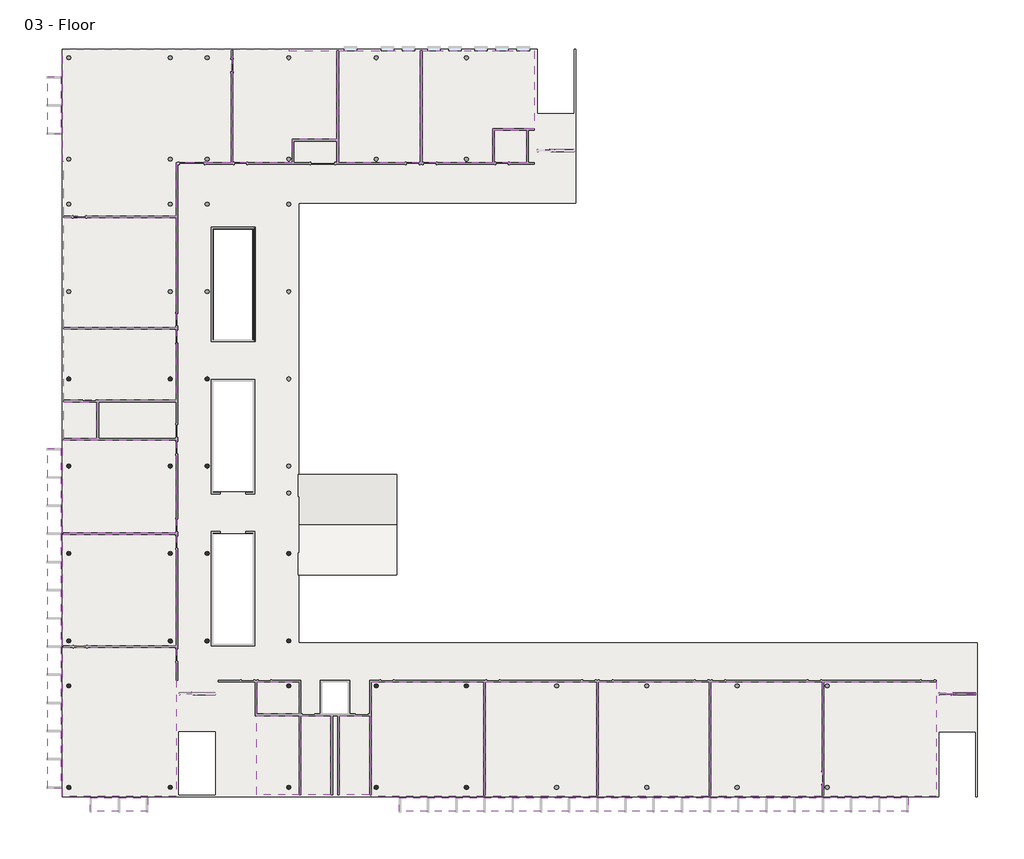
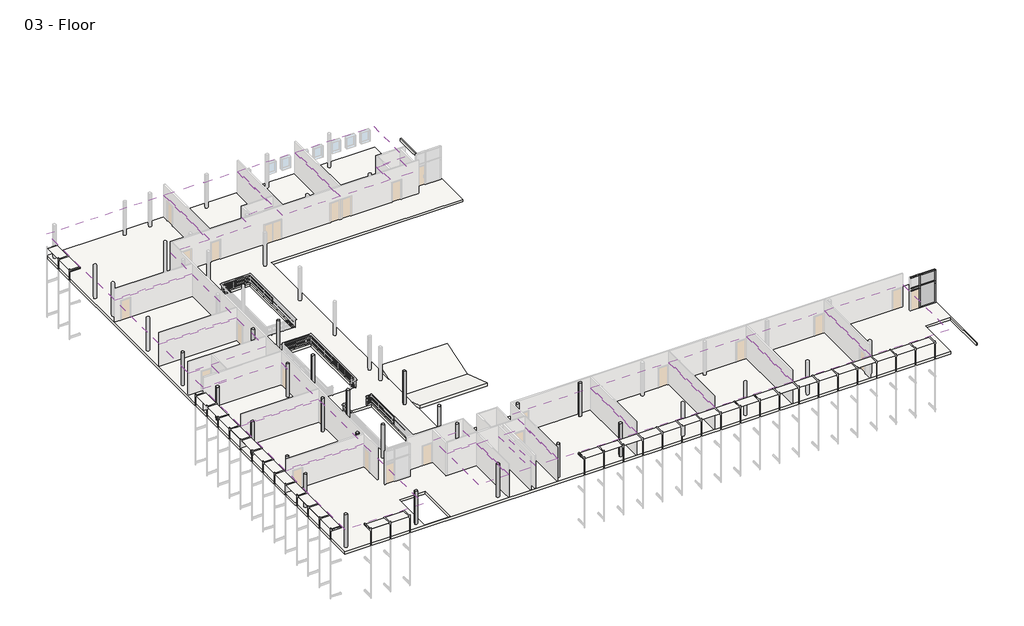
# One storey, part 3 of 4: 23 columns, 20 coverings, 14 members, 5 slabs, 2 plates, 1 roof.
"""IFC4 building model written with IfcOpenShell, lengths in millimetres."""

import ifcopenshell
import ifcopenshell.guid

model = None  # the IFC model being written
_history = None  # IfcOwnerHistory: only IFC2X3 demands one
_inside = {}  # id of a spatial element -> (the spatial element, [elements in it])
_under = {}  # id of a project, library or spatial element -> (it, [spatial elements below it])
_declared = {}  # id of a project -> (the project, [libraries it declares])
_typed = {}  # id of a type object -> (the type object, [elements of that type])
_made_of = {}  # id of a material, layer set ... -> (it, [elements and type objects made of it])


def new_model(schema):
    """Start an empty IFC model of exactly this schema.

    Asked for "IFC4X3", IfcOpenShell would pick the latest addendum, in which some entities
    have other attributes; the version numbers below select the first issue.
    IFC2X3 requires an IfcOwnerHistory on every rooted entity: one is made here for all.
    """
    global model, _history
    if schema == "IFC4X3":
        model = ifcopenshell.file(schema_version=(4, 3, 0, 0))
    else:
        model = ifcopenshell.file(schema=schema)
    _inside.clear()
    _under.clear()
    _declared.clear()
    _typed.clear()
    _made_of.clear()
    _history = None
    if model.schema == "IFC2X3":
        org = make("IfcOrganization", Name="unknown")
        user = make(
            "IfcPersonAndOrganization",
            ThePerson=make("IfcPerson", FamilyName="unknown"),
            TheOrganization=org,
        )
        app = make(
            "IfcApplication",
            ApplicationDeveloper=org,
            Version="unknown",
            ApplicationFullName="unknown",
            ApplicationIdentifier="unknown",
        )
        _history = make(
            "IfcOwnerHistory",
            OwningUser=user,
            OwningApplication=app,
            ChangeAction="ADDED",
            CreationDate=0,
        )
    return model


def make(cls, **values):
    """One entity of the class cls with the attributes given. An attribute that is None is left unset."""
    return model.create_entity(
        cls, **{name: value for name, value in values.items() if value is not None}
    )


def rooted(cls, **values):
    """An entity with a GlobalId (a new one), such as an element, a storey or a relation."""
    return make(cls, GlobalId=ifcopenshell.guid.new(), OwnerHistory=_history, **values)


def si_unit(unit_type, name, prefix=None):
    """IfcSIUnit, for example si_unit("LENGTHUNIT", "METRE", prefix="MILLI")."""
    return make("IfcSIUnit", UnitType=unit_type, Prefix=prefix, Name=name)


def assignment(units):
    """IfcUnitAssignment: the units of a project."""
    return None if units is None else make("IfcUnitAssignment", Units=units)


def point(xyz):
    """IfcCartesianPoint."""
    return None if xyz is None else make("IfcCartesianPoint", Coordinates=xyz)


def direction(xyz):
    """IfcDirection."""
    return None if xyz is None else make("IfcDirection", DirectionRatios=xyz)


def frame(location, z_axis=None, x_axis=None):
    """IfcAxis2Placement3D, a coordinate frame: its origin and axes. An axis left out is left unset."""
    return make(
        "IfcAxis2Placement3D",
        Location=point(location),
        Axis=direction(z_axis),
        RefDirection=direction(x_axis),
    )


def frame_2d(location, x_axis=None):
    """IfcAxis2Placement2D, a coordinate frame in the plane: its origin and x axis."""
    return make(
        "IfcAxis2Placement2D", Location=point(location), RefDirection=direction(x_axis)
    )


def origin():
    """The frame at (0, 0, 0) with its axes left unset."""
    return frame((0.0, 0.0, 0.0))


def place(relative_to, where):
    """IfcLocalPlacement: puts the frame where relative to a parent placement (None: the world)."""
    return make(
        "IfcLocalPlacement", PlacementRelTo=relative_to, RelativePlacement=where
    )


def context(
    kind, dimensions, precision=None, world=None, true_north=None, identifier=None
):
    """IfcGeometricRepresentationContext, for example the 3D "Model" context."""
    return make(
        "IfcGeometricRepresentationContext",
        ContextIdentifier=identifier,
        ContextType=kind,
        CoordinateSpaceDimension=dimensions,
        Precision=precision,
        WorldCoordinateSystem=world,
        TrueNorth=true_north,
    )


def project(units=None, contexts=None):
    """IfcProject with its units and contexts."""
    return rooted(
        "IfcProject",
        Name="project",
        RepresentationContexts=contexts,
        UnitsInContext=assignment(units),
    )


def spatial(cls, under=None, at=None, **own):
    """A site, building, storey or space (cls), placed at a placement, below another one or the project."""
    s = rooted(cls, ObjectPlacement=at, **own)
    if under is not None:
        _under.setdefault(under.id(), (under, []))[1].append(s)
    return s


def polyline(points):
    """IfcPolyline through the points."""
    return make("IfcPolyline", Points=[point(p) for p in points])


def circle_curve(where, radius):
    """IfcCircle in the frame where."""
    return make("IfcCircle", Position=where, Radius=radius)


def trimmed(basis, trim1, trim2, sense, master):
    """IfcTrimmedCurve: the piece of a basis curve between two trims."""
    return make(
        "IfcTrimmedCurve",
        BasisCurve=basis,
        Trim1=trim1,
        Trim2=trim2,
        SenseAgreement=sense,
        MasterRepresentation=master,
    )


def segment(curve, same_sense, transition):
    """IfcCompositeCurveSegment."""
    return make(
        "IfcCompositeCurveSegment",
        Transition=transition,
        SameSense=same_sense,
        ParentCurve=curve,
    )


def composite_curve(segments, self_intersect=None):
    """IfcCompositeCurve: segments joined end to end."""
    return make("IfcCompositeCurve", Segments=segments, SelfIntersect=self_intersect)


def outline(outer, holes=None, kind="AREA"):
    """IfcArbitraryClosedProfileDef: a profile drawn as a closed curve; with holes, ...WithVoids."""
    if holes is None:
        return make("IfcArbitraryClosedProfileDef", ProfileType=kind, OuterCurve=outer)
    return make(
        "IfcArbitraryProfileDefWithVoids",
        ProfileType=kind,
        OuterCurve=outer,
        InnerCurves=holes,
    )


def extrude(swept, where, along, depth):
    """IfcExtrudedAreaSolid: the profile swept, set in the frame where, extruded along a direction by depth."""
    return make(
        "IfcExtrudedAreaSolid",
        SweptArea=swept,
        Position=where,
        ExtrudedDirection=direction(along),
        Depth=depth,
    )


def shape(context_of_items, identifier, shape_type, items):
    """IfcShapeRepresentation: the items that make up one representation, for example the "Body"."""
    return make(
        "IfcShapeRepresentation",
        ContextOfItems=context_of_items,
        RepresentationIdentifier=identifier,
        RepresentationType=shape_type,
        Items=items,
    )


def source(mapping_origin, context_of_items, identifier, shape_type, items):
    """IfcRepresentationMap: a shape defined once, which mapped items show again and again."""
    return make(
        "IfcRepresentationMap",
        MappingOrigin=mapping_origin,
        MappedRepresentation=shape(context_of_items, identifier, shape_type, items),
    )


def transform(
    local_origin,
    x_axis=None,
    y_axis=None,
    z_axis=None,
    scale=None,
    scale2=None,
    scale3=None,
    uniform=True,
):
    """IfcCartesianTransformationOperator3D, or its non-uniform kind. x_axis, y_axis, z_axis: its Axis1, 2, 3."""
    if uniform:
        return make(
            "IfcCartesianTransformationOperator3D",
            Axis1=direction(x_axis),
            Axis2=direction(y_axis),
            LocalOrigin=point(local_origin),
            Scale=scale,
            Axis3=direction(z_axis),
        )
    return make(
        "IfcCartesianTransformationOperator3DnonUniform",
        Axis1=direction(x_axis),
        Axis2=direction(y_axis),
        LocalOrigin=point(local_origin),
        Scale=scale,
        Axis3=direction(z_axis),
        Scale2=scale2,
        Scale3=scale3,
    )


def mapped(mapping_source, mapping_target):
    """IfcMappedItem: shows the shape of a source again, moved by a transform."""
    return make(
        "IfcMappedItem", MappingSource=mapping_source, MappingTarget=mapping_target
    )


def made_of(thing, what):
    """Note that an element or type object is made of a material, layer set ...; save() writes the relation."""
    if what is not None:
        _made_of.setdefault(what.id(), (what, []))[1].append(thing)
    return thing


def element(
    cls,
    number,
    at=None,
    inside=None,
    cuts=None,
    type_object=None,
    material=None,
    context=None,
    identifier="Body",
    shape_type=None,
    held_by="IfcProductDefinitionShape",
    body=None,
    shapes=None,
    **own,
):
    """One element of the class cls, such as IfcWall. Its Tag is "e" and its number.

    at: its placement. inside: the storey or other place that contains it. cuts: it is an
    opening in that element (IfcRelVoidsElement). A single representation is given by context,
    identifier, shape_type and body (its items); several are given by shapes. held_by: the class
    of the entity that holds the representations. save() writes the other relations.
    """
    e = rooted(cls, Tag="e%d" % number, ObjectPlacement=at, **own)
    if body is not None:
        shapes = [shape(context, identifier, shape_type, body)]
    if shapes is not None:
        e.Representation = make(held_by, Representations=shapes)
    if inside is not None:
        _inside.setdefault(inside.id(), (inside, []))[1].append(e)
    if cuts is not None:
        rooted(
            "IfcRelVoidsElement", RelatingBuildingElement=cuts, RelatedOpeningElement=e
        )
    if type_object is not None:
        _typed.setdefault(type_object.id(), (type_object, []))[1].append(e)
    return made_of(e, material)


def aggregate(whole, parts):
    """IfcRelAggregates: a whole, such as a stair, and the parts it consists of."""
    return rooted("IfcRelAggregates", RelatingObject=whole, RelatedObjects=parts)


def save(model, path):
    """Write the relations noted so far, then the file.

    IfcRelAggregates (storeys below a building ...), IfcRelContainedInSpatialStructure (elements
    in a storey), IfcRelDefinesByType, IfcRelAssociatesMaterial and IfcRelDeclares: one each for
    every whole, place, type object, material and project.
    """
    for whole, parts in _under.values():
        aggregate(whole, parts)
    for where, things in _inside.values():
        rooted(
            "IfcRelContainedInSpatialStructure",
            RelatedElements=things,
            RelatingStructure=where,
        )
    for kind, things in _typed.values():
        rooted("IfcRelDefinesByType", RelatedObjects=things, RelatingType=kind)
    for what, things in _made_of.values():
        rooted("IfcRelAssociatesMaterial", RelatedObjects=things, RelatingMaterial=what)
    for by, libraries in _declared.values():
        rooted("IfcRelDeclares", RelatingContext=by, RelatedDefinitions=libraries)
    model.write(path)


def member_2b49869a(model_context):
    return source(origin(), model_context, "Body", "SweptSolid", [
        extrude(outline(polyline([(31.75, 63.5), (31.75, -63.5), (-31.75, -63.5), (-31.75, 63.5), (31.75, 63.5)])), frame((0.0, 0.0, -1219.2), z_axis=(0.0, 0.0, 1.0), x_axis=(1.0, 0.0, 0.0)), (0.0, 0.0, 1.0), 1219.2),
    ])


def member_75074519(model_context):
    return source(origin(), model_context, "Body", "SweptSolid", [
        extrude(outline(polyline([(0.0, 63.5), (0.0, -63.5), (-63.5, -63.5), (-63.5, 63.5), (0.0, 63.5)])), frame((0.0, 0.0, -1219.2), z_axis=(0.0, 0.0, 1.0), x_axis=(1.0, 0.0, 0.0)), (0.0, 0.0, 1.0), 1219.2),
    ])


def member_410c6227(model_context):
    return source(origin(), model_context, "Body", "SweptSolid", [
        extrude(outline(polyline([(31.75, 63.5), (31.75, -63.5), (-31.75, -63.5), (-31.75, 63.5), (31.75, 63.5)])), frame((0.0, 0.0, -914.4), z_axis=(0.0, 0.0, 1.0), x_axis=(1.0, 0.0, 0.0)), (0.0, 0.0, 1.0), 914.4),
    ])


def member_73c23c35(model_context):
    return source(origin(), model_context, "Body", "SweptSolid", [
        extrude(outline(polyline([(0.0, 63.5), (0.0, -63.5), (-63.5, -63.5), (-63.5, 63.5), (0.0, 63.5)])), frame((0.0, 0.0, -914.4), z_axis=(0.0, 0.0, 1.0), x_axis=(1.0, 0.0, 0.0)), (0.0, 0.0, 1.0), 914.4),
    ])


def member_6186cc23(model_context):
    return source(origin(), model_context, "Body", "SweptSolid", [
        extrude(outline(polyline([(31.75, 63.5), (31.75, -63.5), (-31.75, -63.5), (-31.75, 63.5), (31.75, 63.5)])), frame((0.0, 0.0, -2165.35), z_axis=(0.0, 0.0, 1.0), x_axis=(1.0, 0.0, 0.0)), (0.0, 0.0, 1.0), 2165.35),
    ])


def member_5d67b9fc(model_context):
    return source(origin(), model_context, "Body", "SweptSolid", [
        extrude(outline(polyline([(31.75, 63.5), (31.75, -63.5), (-31.75, -63.5), (-31.75, 63.5), (31.75, 63.5)])), frame((0.0, 0.0, -273.05), z_axis=(0.0, 0.0, 1.0), x_axis=(1.0, 0.0, 0.0)), (0.0, 0.0, 1.0), 273.05),
    ])


def member_a50b3cda(model_context):
    return source(origin(), model_context, "Body", "SweptSolid", [
        extrude(outline(polyline([(0.0, 63.5), (0.0, -63.5), (-63.5, -63.5), (-63.5, 63.5), (0.0, 63.5)])), frame((0.0, 0.0, -2165.35), z_axis=(0.0, 0.0, 1.0), x_axis=(1.0, 0.0, 0.0)), (0.0, 0.0, 1.0), 2165.35),
    ])


def member_c327c56d(model_context):
    return source(origin(), model_context, "Body", "SweptSolid", [
        extrude(outline(polyline([(0.0, 63.5), (0.0, -63.5), (-63.5, -63.5), (-63.5, 63.5), (0.0, 63.5)])), frame((0.0, 0.0, -273.05), z_axis=(0.0, 0.0, 1.0), x_axis=(1.0, 0.0, 0.0)), (0.0, 0.0, 1.0), 273.05),
    ])


def member_6c34f49c(model_context):
    return source(origin(), model_context, "Body", "SweptSolid", [
        extrude(outline(polyline([(0.0, 63.5), (0.0, -63.5), (-63.5, -63.5), (-63.5, 63.5), (0.0, 63.5)])), frame((0.0, 0.0, -285.75), z_axis=(0.0, 0.0, 1.0), x_axis=(1.0, 0.0, 0.0)), (0.0, 0.0, 1.0), 285.75),
    ])


def member_dff87739(model_context):
    return source(origin(), model_context, "Body", "SweptSolid", [
        extrude(outline(polyline([(31.75, 63.5), (31.75, -63.5), (-31.75, -63.5), (-31.75, 63.5), (31.75, 63.5)])), frame((0.0, 0.0, -285.75), z_axis=(0.0, 0.0, 1.0), x_axis=(1.0, 0.0, 0.0)), (0.0, 0.0, 1.0), 285.75),
    ])


def member_76223ac8(model_context):
    return source(origin(), model_context, "Body", "SweptSolid", [
        extrude(outline(polyline([(31.75, 63.5), (31.75, -63.5), (-31.75, -63.5), (-31.75, 63.5), (31.75, 63.5)])), frame((0.0, 0.0, -1263.65), z_axis=(0.0, 0.0, 1.0), x_axis=(1.0, 0.0, 0.0)), (0.0, 0.0, 1.0), 1263.65),
    ])


def member_e7b2e991(model_context):
    return source(origin(), model_context, "Body", "SweptSolid", [
        extrude(outline(polyline([(0.0, 63.5), (0.0, -63.5), (-63.5, -63.5), (-63.5, 63.5), (0.0, 63.5)])), frame((0.0, 0.0, -1263.65), z_axis=(0.0, 0.0, 1.0), x_axis=(1.0, 0.0, 0.0)), (0.0, 0.0, 1.0), 1263.65),
    ])


def system_panel_glazed_00df446d(model_context):
    return source(origin(), model_context, "Body", "SweptSolid", [
        extrude(outline(polyline([(0.0, -774.7), (0.0, -488.95), (0.0, 774.7), (2101.85, 774.7), (2343.15, 774.7), (2343.15, -488.95), (2343.15, -774.7), (2101.85, -774.7), (0.0, -774.7)])), frame((0.0, 19.05, 0.0), z_axis=(0.0, 1.0, 0.0), x_axis=(0.0, 0.0, 1.0)), (0.0, 0.0, 1.0), 25.4),
    ])


def system_panel_glazed_835a6d4f(model_context):
    return source(origin(), model_context, "Body", "SweptSolid", [
        extrude(outline(polyline([(0.0, -774.7), (0.0, -488.95), (0.0, 774.7), (1123.95, 774.7), (1123.95, -488.95), (1123.95, -774.7), (0.0, -774.7)])), frame((0.0, 19.05, 0.0), z_axis=(0.0, 1.0, 0.0), x_axis=(0.0, 0.0, 1.0)), (0.0, 0.0, 1.0), 25.4),
    ])


model = new_model("IFC4")

# Units and contexts
model_context = context("Model", 3, world=origin())
ifc_project = project(units=[si_unit("LENGTHUNIT", "METRE", prefix="MILLI")], contexts=[model_context])

# Site, building, storey
site = spatial("IfcSite", under=ifc_project)
building = spatial("IfcBuilding", under=site)
storey = spatial("IfcBuildingStorey", under=building, Name="03 - Floor", Elevation=7315.2)

# Columns
placement = place(None, origin())
element("IfcColumn", 1, ObjectType="Concrete-Round-Column : 12\"", at=placement, inside=storey, context=model_context, shape_type="SweptSolid", body=[
    extrude(outline(composite_curve([segment(trimmed(circle_curve(frame_2d((635.9207476, 30064.0)), 152.4), [point((788.3207476, 30064.0))], [point((483.5207476, 30064.0))], False, "CARTESIAN"), True, "CONTINUOUS"), segment(trimmed(circle_curve(frame_2d((635.9207476, 30064.0)), 152.4), [point((483.5207476, 30064.0))], [point((788.3207476, 30064.0))], False, "CARTESIAN"), True, "CONTINUOUS")], self_intersect=False)), frame((0.0, 0.0, 7315.2), z_axis=(0.0, 0.0, 1.0), x_axis=(1.0, 0.0, 0.0)), (0.0, 0.0, 1.0), 3657.6),
])
element("IfcColumn", 2, ObjectType="Concrete-Round-Column : 12\"", at=placement, inside=storey, context=model_context, shape_type="SweptSolid", body=[
    extrude(outline(composite_curve([segment(trimmed(circle_curve(frame_2d((635.9207476, 23764.8)), 152.4), [point((788.3207476, 23764.8))], [point((483.5207476, 23764.8))], False, "CARTESIAN"), True, "CONTINUOUS"), segment(trimmed(circle_curve(frame_2d((635.9207476, 23764.8)), 152.4), [point((483.5207476, 23764.8))], [point((788.3207476, 23764.8))], False, "CARTESIAN"), True, "CONTINUOUS")], self_intersect=False)), frame((0.0, 0.0, 7315.2), z_axis=(0.0, 0.0, 1.0), x_axis=(1.0, 0.0, 0.0)), (0.0, 0.0, 1.0), 3657.6),
])
element("IfcColumn", 3, ObjectType="Concrete-Round-Column : 12\"", at=placement, inside=storey, context=model_context, shape_type="SweptSolid", body=[
    extrude(outline(composite_curve([segment(trimmed(circle_curve(frame_2d((635.9207476, 17465.6)), 152.4), [point((788.3207476, 17465.6))], [point((483.5207476, 17465.6))], False, "CARTESIAN"), True, "CONTINUOUS"), segment(trimmed(circle_curve(frame_2d((635.9207476, 17465.6)), 152.4), [point((483.5207476, 17465.6))], [point((788.3207476, 17465.6))], False, "CARTESIAN"), True, "CONTINUOUS")], self_intersect=False)), frame((0.0, 0.0, 7315.2), z_axis=(0.0, 0.0, 1.0), x_axis=(1.0, 0.0, 0.0)), (0.0, 0.0, 1.0), 3657.6),
])
element("IfcColumn", 4, ObjectType="Concrete-Round-Column : 12\"", at=placement, inside=storey, context=model_context, shape_type="SweptSolid", body=[
    extrude(outline(composite_curve([segment(trimmed(circle_curve(frame_2d((635.9207476, 11166.4)), 152.4), [point((788.3207476, 11166.4))], [point((483.5207476, 11166.4))], False, "CARTESIAN"), True, "CONTINUOUS"), segment(trimmed(circle_curve(frame_2d((635.9207476, 11166.4)), 152.4), [point((483.5207476, 11166.4))], [point((788.3207476, 11166.4))], False, "CARTESIAN"), True, "CONTINUOUS")], self_intersect=False)), frame((0.0, 0.0, 7315.2), z_axis=(0.0, 0.0, 1.0), x_axis=(1.0, 0.0, 0.0)), (0.0, 0.0, 1.0), 3657.6),
])
element("IfcColumn", 5, ObjectType="Concrete-Round-Column : 12\"", at=placement, inside=storey, context=model_context, shape_type="SweptSolid", body=[
    extrude(outline(composite_curve([segment(trimmed(circle_curve(frame_2d((635.9207476, 7915.2)), 152.4), [point((788.3207476, 7915.2))], [point((483.5207476, 7915.2))], False, "CARTESIAN"), True, "CONTINUOUS"), segment(trimmed(circle_curve(frame_2d((635.9207476, 7915.2)), 152.4), [point((483.5207476, 7915.2))], [point((788.3207476, 7915.2))], False, "CARTESIAN"), True, "CONTINUOUS")], self_intersect=False)), frame((0.0, 0.0, 7315.2), z_axis=(0.0, 0.0, 1.0), x_axis=(1.0, 0.0, 0.0)), (0.0, 0.0, 1.0), 3657.6),
])
element("IfcColumn", 6, ObjectType="Concrete-Round-Column : 12\"", at=placement, inside=storey, context=model_context, shape_type="SweptSolid", body=[
    extrude(outline(composite_curve([segment(trimmed(circle_curve(frame_2d((635.9207476, 600.0)), 152.4), [point((788.3207476, 600.0))], [point((483.5207476, 600.0))], False, "CARTESIAN"), True, "CONTINUOUS"), segment(trimmed(circle_curve(frame_2d((635.9207476, 600.0)), 152.4), [point((483.5207476, 600.0))], [point((788.3207476, 600.0))], False, "CARTESIAN"), True, "CONTINUOUS")], self_intersect=False)), frame((0.0, 0.0, 7315.2), z_axis=(0.0, 0.0, 1.0), x_axis=(1.0, 0.0, 0.0)), (0.0, 0.0, 1.0), 3657.6),
])
element("IfcColumn", 7, ObjectType="Concrete-Round-Column : 12\"", at=placement, inside=storey, context=model_context, shape_type="SweptSolid", body=[
    extrude(outline(composite_curve([segment(trimmed(circle_curve(frame_2d((10592.7207476, 30064.0)), 152.4), [point((10745.1207476, 30064.0))], [point((10440.3207476, 30064.0))], False, "CARTESIAN"), True, "CONTINUOUS"), segment(trimmed(circle_curve(frame_2d((10592.7207476, 30064.0)), 152.4), [point((10440.3207476, 30064.0))], [point((10745.1207476, 30064.0))], False, "CARTESIAN"), True, "CONTINUOUS")], self_intersect=False)), frame((0.0, 0.0, 7315.2), z_axis=(0.0, 0.0, 1.0), x_axis=(1.0, 0.0, 0.0)), (0.0, 0.0, 1.0), 3657.6),
])
element("IfcColumn", 8, ObjectType="Concrete-Round-Column : 12\"", at=placement, inside=storey, context=model_context, shape_type="SweptSolid", body=[
    extrude(outline(composite_curve([segment(trimmed(circle_curve(frame_2d((10592.7207476, 23764.8)), 152.4), [point((10745.1207476, 23764.8))], [point((10440.3207476, 23764.8))], False, "CARTESIAN"), True, "CONTINUOUS"), segment(trimmed(circle_curve(frame_2d((10592.7207476, 23764.8)), 152.4), [point((10440.3207476, 23764.8))], [point((10745.1207476, 23764.8))], False, "CARTESIAN"), True, "CONTINUOUS")], self_intersect=False)), frame((0.0, 0.0, 7315.2), z_axis=(0.0, 0.0, 1.0), x_axis=(1.0, 0.0, 0.0)), (0.0, 0.0, 1.0), 3657.6),
])
element("IfcColumn", 9, ObjectType="Concrete-Round-Column : 12\"", at=placement, inside=storey, context=model_context, shape_type="SweptSolid", body=[
    extrude(outline(composite_curve([segment(trimmed(circle_curve(frame_2d((10592.7207476, 17465.6)), 152.4), [point((10745.1207476, 17465.6))], [point((10440.3207476, 17465.6))], False, "CARTESIAN"), True, "CONTINUOUS"), segment(trimmed(circle_curve(frame_2d((10592.7207476, 17465.6)), 152.4), [point((10440.3207476, 17465.6))], [point((10745.1207476, 17465.6))], False, "CARTESIAN"), True, "CONTINUOUS")], self_intersect=False)), frame((0.0, 0.0, 7315.2), z_axis=(0.0, 0.0, 1.0), x_axis=(1.0, 0.0, 0.0)), (0.0, 0.0, 1.0), 3657.6),
])
element("IfcColumn", 10, ObjectType="Concrete-Round-Column : 12\"", at=placement, inside=storey, context=model_context, shape_type="SweptSolid", body=[
    extrude(outline(composite_curve([segment(trimmed(circle_curve(frame_2d((10592.7207476, 11166.4)), 152.4), [point((10745.1207476, 11166.4))], [point((10440.3207476, 11166.4))], False, "CARTESIAN"), True, "CONTINUOUS"), segment(trimmed(circle_curve(frame_2d((10592.7207476, 11166.4)), 152.4), [point((10440.3207476, 11166.4))], [point((10745.1207476, 11166.4))], False, "CARTESIAN"), True, "CONTINUOUS")], self_intersect=False)), frame((0.0, 0.0, 7315.2), z_axis=(0.0, 0.0, 1.0), x_axis=(1.0, 0.0, 0.0)), (0.0, 0.0, 1.0), 3657.6),
])
element("IfcColumn", 11, ObjectType="Concrete-Round-Column : 12\"", at=placement, inside=storey, context=model_context, shape_type="SweptSolid", body=[
    extrude(outline(composite_curve([segment(trimmed(circle_curve(frame_2d((16485.5207476, 17465.6)), 152.4), [point((16637.9207476, 17465.6))], [point((16333.1207476, 17465.6))], False, "CARTESIAN"), True, "CONTINUOUS"), segment(trimmed(circle_curve(frame_2d((16485.5207476, 17465.6)), 152.4), [point((16333.1207476, 17465.6))], [point((16637.9207476, 17465.6))], False, "CARTESIAN"), True, "CONTINUOUS")], self_intersect=False)), frame((0.0, 0.0, 7315.2), z_axis=(0.0, 0.0, 1.0), x_axis=(1.0, 0.0, 0.0)), (0.0, 0.0, 1.0), 3657.6),
])
element("IfcColumn", 12, ObjectType="Concrete-Round-Column : 12\"", at=placement, inside=storey, context=model_context, shape_type="SweptSolid", body=[
    extrude(outline(composite_curve([segment(trimmed(circle_curve(frame_2d((16485.5207476, 11166.4)), 152.4), [point((16637.9207476, 11166.4))], [point((16333.1207476, 11166.4))], False, "CARTESIAN"), True, "CONTINUOUS"), segment(trimmed(circle_curve(frame_2d((16485.5207476, 11166.4)), 152.4), [point((16333.1207476, 11166.4))], [point((16637.9207476, 11166.4))], False, "CARTESIAN"), True, "CONTINUOUS")], self_intersect=False)), frame((0.0, 0.0, 7315.2), z_axis=(0.0, 0.0, 1.0), x_axis=(1.0, 0.0, 0.0)), (0.0, 0.0, 1.0), 3657.6),
])
element("IfcColumn", 13, ObjectType="Concrete-Round-Column : 12\"", at=placement, inside=storey, context=model_context, shape_type="SweptSolid", body=[
    extrude(outline(composite_curve([segment(trimmed(circle_curve(frame_2d((16485.5207476, 7915.2)), 152.4), [point((16637.9207476, 7915.2))], [point((16333.1207476, 7915.2))], False, "CARTESIAN"), True, "CONTINUOUS"), segment(trimmed(circle_curve(frame_2d((16485.5207476, 7915.2)), 152.4), [point((16333.1207476, 7915.2))], [point((16637.9207476, 7915.2))], False, "CARTESIAN"), True, "CONTINUOUS")], self_intersect=False)), frame((0.0, 0.0, 7315.2), z_axis=(0.0, 0.0, 1.0), x_axis=(1.0, 0.0, 0.0)), (0.0, 0.0, 1.0), 3657.6),
])
element("IfcColumn", 14, ObjectType="Concrete-Round-Column : 12\"", at=placement, inside=storey, context=model_context, shape_type="SweptSolid", body=[
    extrude(outline(composite_curve([segment(trimmed(circle_curve(frame_2d((16485.5207476, 600.0)), 152.4), [point((16637.9207476, 600.0))], [point((16333.1207476, 600.0))], False, "CARTESIAN"), True, "CONTINUOUS"), segment(trimmed(circle_curve(frame_2d((16485.5207476, 600.0)), 152.4), [point((16333.1207476, 600.0))], [point((16637.9207476, 600.0))], False, "CARTESIAN"), True, "CONTINUOUS")], self_intersect=False)), frame((0.0, 0.0, 7315.2), z_axis=(0.0, 0.0, 1.0), x_axis=(1.0, 0.0, 0.0)), (0.0, 0.0, 1.0), 3657.6),
])
element("IfcColumn", 15, ObjectType="Concrete-Round-Column : 12\"", at=placement, inside=storey, context=model_context, shape_type="SweptSolid", body=[
    extrude(outline(composite_curve([segment(trimmed(circle_curve(frame_2d((22784.7207476, 7915.2)), 152.4), [point((22937.1207476, 7915.2))], [point((22632.3207476, 7915.2))], False, "CARTESIAN"), True, "CONTINUOUS"), segment(trimmed(circle_curve(frame_2d((22784.7207476, 7915.2)), 152.4), [point((22632.3207476, 7915.2))], [point((22937.1207476, 7915.2))], False, "CARTESIAN"), True, "CONTINUOUS")], self_intersect=False)), frame((0.0, 0.0, 7315.2), z_axis=(0.0, 0.0, 1.0), x_axis=(1.0, 0.0, 0.0)), (0.0, 0.0, 1.0), 3657.6),
])
element("IfcColumn", 16, ObjectType="Concrete-Round-Column : 12\"", at=placement, inside=storey, context=model_context, shape_type="SweptSolid", body=[
    extrude(outline(composite_curve([segment(trimmed(circle_curve(frame_2d((22784.7207476, 600.0)), 152.4), [point((22937.1207476, 600.0))], [point((22632.3207476, 600.0))], False, "CARTESIAN"), True, "CONTINUOUS"), segment(trimmed(circle_curve(frame_2d((22784.7207476, 600.0)), 152.4), [point((22632.3207476, 600.0))], [point((22937.1207476, 600.0))], False, "CARTESIAN"), True, "CONTINUOUS")], self_intersect=False)), frame((0.0, 0.0, 7315.2), z_axis=(0.0, 0.0, 1.0), x_axis=(1.0, 0.0, 0.0)), (0.0, 0.0, 1.0), 3657.6),
])
element("IfcColumn", 17, ObjectType="Concrete-Round-Column : 12\"", at=placement, inside=storey, context=model_context, shape_type="SweptSolid", body=[
    extrude(outline(composite_curve([segment(trimmed(circle_curve(frame_2d((29287.1207476, 7915.2)), 152.4), [point((29439.5207476, 7915.2))], [point((29134.7207476, 7915.2))], False, "CARTESIAN"), True, "CONTINUOUS"), segment(trimmed(circle_curve(frame_2d((29287.1207476, 7915.2)), 152.4), [point((29134.7207476, 7915.2))], [point((29439.5207476, 7915.2))], False, "CARTESIAN"), True, "CONTINUOUS")], self_intersect=False)), frame((0.0, 0.0, 7315.2), z_axis=(0.0, 0.0, 1.0), x_axis=(1.0, 0.0, 0.0)), (0.0, 0.0, 1.0), 3657.6),
])
element("IfcColumn", 18, ObjectType="Concrete-Round-Column : 12\"", at=placement, inside=storey, context=model_context, shape_type="SweptSolid", body=[
    extrude(outline(composite_curve([segment(trimmed(circle_curve(frame_2d((29287.1207476, 600.0)), 152.4), [point((29439.5207476, 600.0))], [point((29134.7207476, 600.0))], False, "CARTESIAN"), True, "CONTINUOUS"), segment(trimmed(circle_curve(frame_2d((29287.1207476, 600.0)), 152.4), [point((29134.7207476, 600.0))], [point((29439.5207476, 600.0))], False, "CARTESIAN"), True, "CONTINUOUS")], self_intersect=False)), frame((0.0, 0.0, 7315.2), z_axis=(0.0, 0.0, 1.0), x_axis=(1.0, 0.0, 0.0)), (0.0, 0.0, 1.0), 3657.6),
])
element("IfcColumn", 19, ObjectType="Concrete-Round-Column : 12\"", at=placement, inside=storey, context=model_context, shape_type="SweptSolid", body=[
    extrude(outline(composite_curve([segment(trimmed(circle_curve(frame_2d((7951.1207476, 30064.0)), 152.4), [point((8103.5207476, 30064.0))], [point((7798.7207476, 30064.0))], False, "CARTESIAN"), True, "CONTINUOUS"), segment(trimmed(circle_curve(frame_2d((7951.1207476, 30064.0)), 152.4), [point((7798.7207476, 30064.0))], [point((8103.5207476, 30064.0))], False, "CARTESIAN"), True, "CONTINUOUS")], self_intersect=False)), frame((0.0, 0.0, 7315.2), z_axis=(0.0, 0.0, 1.0), x_axis=(1.0, 0.0, 0.0)), (0.0, 0.0, 1.0), 3657.6),
])
element("IfcColumn", 20, ObjectType="Concrete-Round-Column : 12\"", at=placement, inside=storey, context=model_context, shape_type="SweptSolid", body=[
    extrude(outline(composite_curve([segment(trimmed(circle_curve(frame_2d((7951.1207476, 23764.8)), 152.4), [point((8103.5207476, 23764.8))], [point((7798.7207476, 23764.8))], False, "CARTESIAN"), True, "CONTINUOUS"), segment(trimmed(circle_curve(frame_2d((7951.1207476, 23764.8)), 152.4), [point((7798.7207476, 23764.8))], [point((8103.5207476, 23764.8))], False, "CARTESIAN"), True, "CONTINUOUS")], self_intersect=False)), frame((0.0, 0.0, 7315.2), z_axis=(0.0, 0.0, 1.0), x_axis=(1.0, 0.0, 0.0)), (0.0, 0.0, 1.0), 3657.6),
])
element("IfcColumn", 21, ObjectType="Concrete-Round-Column : 12\"", at=placement, inside=storey, context=model_context, shape_type="SweptSolid", body=[
    extrude(outline(composite_curve([segment(trimmed(circle_curve(frame_2d((7951.1207476, 17465.6)), 152.4), [point((8103.5207476, 17465.6))], [point((7798.7207476, 17465.6))], False, "CARTESIAN"), True, "CONTINUOUS"), segment(trimmed(circle_curve(frame_2d((7951.1207476, 17465.6)), 152.4), [point((7798.7207476, 17465.6))], [point((8103.5207476, 17465.6))], False, "CARTESIAN"), True, "CONTINUOUS")], self_intersect=False)), frame((0.0, 0.0, 7315.2), z_axis=(0.0, 0.0, 1.0), x_axis=(1.0, 0.0, 0.0)), (0.0, 0.0, 1.0), 3657.6),
])
element("IfcColumn", 22, ObjectType="Concrete-Round-Column : 12\"", at=placement, inside=storey, context=model_context, shape_type="SweptSolid", body=[
    extrude(outline(composite_curve([segment(trimmed(circle_curve(frame_2d((7951.1207476, 11166.4)), 152.4), [point((8103.5207476, 11166.4))], [point((7798.7207476, 11166.4))], False, "CARTESIAN"), True, "CONTINUOUS"), segment(trimmed(circle_curve(frame_2d((7951.1207476, 11166.4)), 152.4), [point((7798.7207476, 11166.4))], [point((8103.5207476, 11166.4))], False, "CARTESIAN"), True, "CONTINUOUS")], self_intersect=False)), frame((0.0, 0.0, 7315.2), z_axis=(0.0, 0.0, 1.0), x_axis=(1.0, 0.0, 0.0)), (0.0, 0.0, 1.0), 3657.6),
])
element("IfcColumn", 23, ObjectType="Concrete-Round-Column : 12\"", at=placement, inside=storey, context=model_context, shape_type="SweptSolid", body=[
    extrude(outline(composite_curve([segment(trimmed(circle_curve(frame_2d((7951.1207476, 600.0)), 152.4), [point((8103.5207476, 600.0))], [point((7798.7207476, 600.0))], False, "CARTESIAN"), True, "CONTINUOUS"), segment(trimmed(circle_curve(frame_2d((7951.1207476, 600.0)), 152.4), [point((7798.7207476, 600.0))], [point((8103.5207476, 600.0))], False, "CARTESIAN"), True, "CONTINUOUS")], self_intersect=False)), frame((0.0, 0.0, 7315.2), z_axis=(0.0, 0.0, 1.0), x_axis=(1.0, 0.0, 0.0)), (0.0, 0.0, 1.0), 3657.6),
])

# Coverings
element("IfcCovering", 24, ObjectType="2' x 2' ACT System", at=placement, inside=storey, context=model_context, shape_type="SweptSolid", body=[
    extrude(outline(polyline([(26093.0707476, 45659.6), (26093.0707476, 53724.1), (34194.0832476, 53724.1), (34194.0832476, 48104.35), (31198.4707476, 48104.35), (31198.4707476, 45659.6), (26093.0707476, 45659.6)])), frame((0.0, 0.0, 9753.6), z_axis=(0.0, 0.0, 1.0), x_axis=(1.0, 0.0, 0.0)), (0.0, 0.0, 1.0), 57.15),
])
element("IfcCovering", 25, ObjectType="2' x 2' ACT System", at=placement, inside=storey, context=model_context, shape_type="SweptSolid", body=[
    extrude(outline(polyline([(33636.8707476, 45659.6), (31312.7707476, 45659.6), (31312.7707476, 47990.05), (33636.8707476, 47990.05), (33636.8707476, 45659.6)])), frame((0.0, 0.0, 9753.6), z_axis=(0.0, 0.0, 1.0), x_axis=(1.0, 0.0, 0.0)), (0.0, 0.0, 1.0), 57.15),
])
element("IfcCovering", 26, ObjectType="2' x 2' ACT System", at=placement, inside=storey, context=model_context, shape_type="SweptSolid", body=[
    extrude(outline(polyline([(20073.2707476, 45659.6), (20073.2707476, 53724.1), (25978.7707476, 53724.1), (25978.7707476, 45659.6), (20073.2707476, 45659.6)])), frame((0.0, 0.0, 9753.6), z_axis=(0.0, 0.0, 1.0), x_axis=(1.0, 0.0, 0.0)), (0.0, 0.0, 1.0), 57.15),
])
element("IfcCovering", 27, ObjectType="2' x 2' ACT System", at=placement, inside=storey, context=model_context, shape_type="SweptSolid", body=[
    extrude(outline(polyline([(12453.2707476, 53825.7), (16491.8707476, 53825.7), (16491.8707476, 53724.1), (19958.9707476, 53724.1), (19958.9707476, 47338.3500002), (16720.4707476, 47338.3500002), (16720.4707476, 45659.6), (12453.2707476, 45659.6), (12453.2707476, 53825.7)])), frame((0.0, 0.0, 9753.6), z_axis=(0.0, 0.0, 1.0), x_axis=(1.0, 0.0, 0.0)), (0.0, 0.0, 1.0), 57.15),
])
element("IfcCovering", 28, ObjectType="2' x 2' ACT System", at=placement, inside=storey, context=model_context, shape_type="SweptSolid", body=[
    extrude(outline(polyline([(280.3207476, 41805.15), (280.3207476, 45729.45), (178.7207476, 45729.45), (178.7207476, 53825.7), (12338.9707476, 53825.7), (12338.9707476, 45659.6), (8357.5207476, 45659.6), (8357.5207476, 41805.15), (280.3207476, 41805.15)])), frame((0.0, 0.0, 9753.6), z_axis=(0.0, 0.0, 1.0), x_axis=(1.0, 0.0, 0.0)), (0.0, 0.0, 1.0), 57.15),
])
element("IfcCovering", 29, ObjectType="2' x 2' ACT System", at=placement, inside=storey, context=model_context, shape_type="SweptSolid", body=[
    extrude(outline(polyline([(8357.5207476, 33778.75), (280.3207476, 33778.75), (280.3207476, 41690.85), (8357.5207476, 41690.85), (8357.5207476, 33778.75)])), frame((0.0, 0.0, 9753.6), z_axis=(0.0, 0.0, 1.0), x_axis=(1.0, 0.0, 0.0)), (0.0, 0.0, 1.0), 57.15),
])
element("IfcCovering", 30, ObjectType="2' x 2' ACT System", at=placement, inside=storey, context=model_context, shape_type="SweptSolid", body=[
    extrude(outline(polyline([(8357.5207476, 28520.95), (280.3207476, 28520.95), (280.3207476, 33664.45), (8357.5207476, 33664.45), (8357.5207476, 28520.95)])), frame((0.0, 0.0, 9753.6), z_axis=(0.0, 0.0, 1.0), x_axis=(1.0, 0.0, 0.0)), (0.0, 0.0, 1.0), 57.15),
])
element("IfcCovering", 31, ObjectType="2' x 2' ACT System", at=placement, inside=storey, context=model_context, shape_type="SweptSolid", body=[
    extrude(outline(polyline([(8357.5207476, 18945.15), (178.7207476, 18945.15), (178.7207476, 25638.05), (8357.5207476, 25638.05), (8357.5207476, 18945.15)])), frame((0.0, 0.0, 9753.6), z_axis=(0.0, 0.0, 1.0), x_axis=(1.0, 0.0, 0.0)), (0.0, 0.0, 1.0), 57.15),
])
element("IfcCovering", 32, ObjectType="2' x 2' ACT System", at=placement, inside=storey, context=model_context, shape_type="SweptSolid", body=[
    extrude(outline(polyline([(8357.5207476, 10817.15), (178.7207476, 10817.15), (178.7207476, 18830.85), (8357.5207476, 18830.85), (8357.5207476, 10817.15)])), frame((0.0, 0.0, 9753.6), z_axis=(0.0, 0.0, 1.0), x_axis=(1.0, 0.0, 0.0)), (0.0, 0.0, 1.0), 57.15),
])
element("IfcCovering", 33, ObjectType="2' x 2' ACT System", at=placement, inside=storey, context=model_context, shape_type="SweptSolid", body=[
    extrude(outline(polyline([(14180.4707476, 8220.0), (17241.1707476, 8220.0), (17241.1707476, 5889.55), (14180.4707476, 5889.55), (14180.4707476, 8220.0)])), frame((0.0, 0.0, 9753.6), z_axis=(0.0, 0.0, 1.0), x_axis=(1.0, 0.0, 0.0)), (0.0, 0.0, 1.0), 57.15),
])
element("IfcCovering", 34, ObjectType="2' x 2' ACT System", at=placement, inside=storey, context=model_context, shape_type="SweptSolid", body=[
    extrude(outline(polyline([(17241.1707476, 5775.25), (17241.1707476, 53.9), (14180.4707476, 53.9), (14180.4707476, 5775.25), (17241.1707476, 5775.25)])), frame((0.0, 0.0, 9753.6), z_axis=(0.0, 0.0, 1.0), x_axis=(1.0, 0.0, 0.0)), (0.0, 0.0, 1.0), 57.15),
])
element("IfcCovering", 35, ObjectType="2' x 2' ACT System", at=placement, inside=storey, context=model_context, shape_type="SweptSolid", body=[
    extrude(outline(polyline([(19527.1707476, 53.9), (17355.4707476, 53.9), (17355.4707476, 5775.25), (19527.1707476, 5775.25), (19527.1707476, 53.9)])), frame((0.0, 0.0, 9753.6), z_axis=(0.0, 0.0, 1.0), x_axis=(1.0, 0.0, 0.0)), (0.0, 0.0, 1.0), 57.15),
])
element("IfcCovering", 36, ObjectType="2' x 2' ACT System", at=placement, inside=storey, context=model_context, shape_type="SweptSolid", body=[
    extrude(outline(polyline([(22308.4707476, 5775.25), (22308.4707476, 53.9), (20124.0707476, 53.9), (20124.0707476, 5775.25), (22308.4707476, 5775.25)])), frame((0.0, 0.0, 9753.6), z_axis=(0.0, 0.0, 1.0), x_axis=(1.0, 0.0, 0.0)), (0.0, 0.0, 1.0), 57.15),
])
element("IfcCovering", 37, ObjectType="2' x 2' ACT System", at=placement, inside=storey, context=model_context, shape_type="SweptSolid", body=[
    extrude(outline(polyline([(30538.0707476, 8220.0), (30538.0707476, -47.7), (22422.7707476, -47.7), (22422.7707476, 8220.0), (30538.0707476, 8220.0)])), frame((0.0, 0.0, 9753.6), z_axis=(0.0, 0.0, 1.0), x_axis=(1.0, 0.0, 0.0)), (0.0, 0.0, 1.0), 57.15),
])
element("IfcCovering", 38, ObjectType="2' x 2' ACT System", at=placement, inside=storey, context=model_context, shape_type="SweptSolid", body=[
    extrude(outline(polyline([(38666.0707476, 8220.0), (38666.0707476, -47.7), (30652.3707476, -47.7), (30652.3707476, 8220.0), (38666.0707476, 8220.0)])), frame((0.0, 0.0, 9753.6), z_axis=(0.0, 0.0, 1.0), x_axis=(1.0, 0.0, 0.0)), (0.0, 0.0, 1.0), 57.15),
])
element("IfcCovering", 39, ObjectType="2' x 2' ACT System", at=placement, inside=storey, context=model_context, shape_type="SweptSolid", body=[
    extrude(outline(polyline([(46794.0707476, 8220.0), (46794.0707476, -47.7), (38780.3707476, -47.7), (38780.3707476, 8220.0), (46794.0707476, 8220.0)])), frame((0.0, 0.0, 9753.6), z_axis=(0.0, 0.0, 1.0), x_axis=(1.0, 0.0, 0.0)), (0.0, 0.0, 1.0), 57.15),
])
element("IfcCovering", 40, ObjectType="2' x 2' ACT System", at=placement, inside=storey, context=model_context, shape_type="SweptSolid", body=[
    extrude(outline(polyline([(54922.0707476, 8220.0), (54922.0707476, -47.7), (46908.3707476, -47.7), (46908.3707476, 8220.0), (54922.0707476, 8220.0)])), frame((0.0, 0.0, 9753.6), z_axis=(0.0, 0.0, 1.0), x_axis=(1.0, 0.0, 0.0)), (0.0, 0.0, 1.0), 57.15),
])
element("IfcCovering", 41, ObjectType="2' x 2' ACT System", at=placement, inside=storey, context=model_context, shape_type="SweptSolid", body=[
    extrude(outline(polyline([(63137.3832476, 8220.0), (63137.3832476, -47.7), (55036.3707476, -47.7), (55036.3707476, 8220.0), (63137.3832476, 8220.0)])), frame((0.0, 0.0, 9753.6), z_axis=(0.0, 0.0, 1.0), x_axis=(1.0, 0.0, 0.0)), (0.0, 0.0, 1.0), 57.15),
])
element("IfcCovering", 42, ObjectType="2' x 2' ACT System", at=placement, inside=storey, context=model_context, shape_type="SweptSolid", body=[
    extrude(outline(polyline([(8357.5207476, -47.7), (178.7207476, -47.7), (178.7207476, 10702.85), (8357.5207476, 10702.85), (8357.5207476, 8334.3), (8357.5207476, -47.7)])), frame((0.0, 0.0, 9753.6), z_axis=(0.0, 0.0, 1.0), x_axis=(1.0, 0.0, 0.0)), (0.0, 0.0, 1.0), 57.15),
])
element("IfcCovering", 43, ObjectType="2' x 2' ACT System", at=placement, inside=storey, context=model_context, shape_type="SweptSolid", body=[
    extrude(outline(polyline([(2661.5707476, 25752.35), (280.3207476, 25752.35), (280.3207476, 28406.65), (2661.5707476, 28406.65), (2661.5707476, 25752.35)])), frame((0.0, 0.0, 9753.6), z_axis=(0.0, 0.0, 1.0), x_axis=(1.0, 0.0, 0.0)), (0.0, 0.0, 1.0), 57.15),
])

# Members
member_shape = member_2b49869a(model_context)
element("IfcMember", 44, ObjectType="Rectangular Mullion : 2.5\" x 5\" rectangular", at=placement, inside=storey, context=model_context, shape_type="MappedRepresentation", body=[
    mapped(member_shape, transform((64358.1707476, 7356.4, 9753.6), x_axis=(1.0, 0.0, 0.0), y_axis=(0.0, -1.0, 0.0), z_axis=(0.0, 0.0, -1.0))),
])
member_2_shape = member_75074519(model_context)
element("IfcMember", 45, ObjectType="Rectangular Mullion : 2.5\" x 5\" rectangular", at=placement, inside=storey, context=model_context, shape_type="MappedRepresentation", body=[
    mapped(member_2_shape, transform((66002.8207476, 7356.4, 9753.6), x_axis=(1.0, 0.0, 0.0), y_axis=(0.0, -1.0, 0.0), z_axis=(0.0, 0.0, -1.0))),
])
member_3_shape = member_410c6227(model_context)
element("IfcMember", 46, ObjectType="Rectangular Mullion : 2.5\" x 5\" rectangular", at=placement, inside=storey, context=model_context, shape_type="MappedRepresentation", body=[
    mapped(member_3_shape, transform((64326.4207476, 7356.4, 9753.6), x_axis=(0.0, 0.0, 1.0), y_axis=(0.0, -1.0, 0.0), z_axis=(1.0, 0.0, 0.0))),
])
element("IfcMember", 47, ObjectType="Rectangular Mullion : 2.5\" x 5\" rectangular", at=placement, inside=storey, context=model_context, shape_type="MappedRepresentation", body=[
    mapped(member_3_shape, transform((64326.4207476, 7356.4, 9480.55), x_axis=(0.0, 0.0, 1.0), y_axis=(0.0, -1.0, 0.0), z_axis=(1.0, 0.0, 0.0))),
])
member_4_shape = member_73c23c35(model_context)
element("IfcMember", 48, ObjectType="Rectangular Mullion : 2.5\" x 5\" rectangular", at=placement, inside=storey, context=model_context, shape_type="MappedRepresentation", body=[
    mapped(member_4_shape, transform((64326.4207476, 7356.4, 10972.8), x_axis=(0.0, 0.0, 1.0), y_axis=(0.0, -1.0, 0.0), z_axis=(1.0, 0.0, 0.0))),
])
member_5_shape = member_6186cc23(model_context)
element("IfcMember", 49, ObjectType="Rectangular Mullion : 2.5\" x 5\" rectangular", at=placement, inside=storey, context=model_context, shape_type="MappedRepresentation", body=[
    mapped(member_5_shape, transform((64358.1707476, 7356.4, 7315.2), x_axis=(1.0, 0.0, 0.0), y_axis=(0.0, -1.0, 0.0), z_axis=(0.0, 0.0, -1.0))),
])
member_6_shape = member_5d67b9fc(model_context)
element("IfcMember", 50, ObjectType="Rectangular Mullion : 2.5\" x 5\" rectangular", at=placement, inside=storey, context=model_context, shape_type="MappedRepresentation", body=[
    mapped(member_6_shape, transform((64358.1707476, 7356.4, 9480.55), x_axis=(1.0, 0.0, 0.0), y_axis=(0.0, -1.0, 0.0), z_axis=(0.0, 0.0, -1.0))),
])
member_7_shape = member_a50b3cda(model_context)
element("IfcMember", 51, ObjectType="Rectangular Mullion : 2.5\" x 5\" rectangular", at=placement, inside=storey, context=model_context, shape_type="MappedRepresentation", body=[
    mapped(member_7_shape, transform((66002.8207476, 7356.4, 7315.2), x_axis=(1.0, 0.0, 0.0), y_axis=(0.0, -1.0, 0.0), z_axis=(0.0, 0.0, -1.0))),
])
member_8_shape = member_c327c56d(model_context)
element("IfcMember", 52, ObjectType="Rectangular Mullion : 2.5\" x 5\" rectangular", at=placement, inside=storey, context=model_context, shape_type="MappedRepresentation", body=[
    mapped(member_8_shape, transform((66002.8207476, 7356.4, 9480.55), x_axis=(1.0, 0.0, 0.0), y_axis=(0.0, -1.0, 0.0), z_axis=(0.0, 0.0, -1.0))),
])
member_9_shape = member_6c34f49c(model_context)
element("IfcMember", 53, ObjectType="Rectangular Mullion : 2.5\" x 5\" rectangular", at=placement, inside=storey, context=model_context, shape_type="MappedRepresentation", body=[
    mapped(member_9_shape, transform((64389.9207476, 7356.4, 7315.2), x_axis=(0.0, 0.0, -1.0), y_axis=(0.0, -1.0, 0.0), z_axis=(-1.0, 0.0, 0.0))),
])
member_10_shape = member_dff87739(model_context)
element("IfcMember", 54, ObjectType="Rectangular Mullion : 2.5\" x 5\" rectangular", at=placement, inside=storey, context=model_context, shape_type="MappedRepresentation", body=[
    mapped(member_10_shape, transform((64675.6707476, 7356.4, 9753.6), x_axis=(0.0, 0.0, 1.0), y_axis=(0.0, -1.0, 0.0), z_axis=(1.0, 0.0, 0.0))),
])
member_11_shape = member_76223ac8(model_context)
element("IfcMember", 55, ObjectType="Rectangular Mullion : 2.5\" x 5\" rectangular", at=placement, inside=storey, context=model_context, shape_type="MappedRepresentation", body=[
    mapped(member_11_shape, transform((65939.3207476, 7356.4, 9753.6), x_axis=(0.0, 0.0, 1.0), y_axis=(0.0, -1.0, 0.0), z_axis=(1.0, 0.0, 0.0))),
])
member_12_shape = member_e7b2e991(model_context)
element("IfcMember", 56, ObjectType="Rectangular Mullion : 2.5\" x 5\" rectangular", at=placement, inside=storey, context=model_context, shape_type="MappedRepresentation", body=[
    mapped(member_12_shape, transform((65939.3207476, 7356.4, 10972.8), x_axis=(0.0, 0.0, 1.0), y_axis=(0.0, -1.0, 0.0), z_axis=(1.0, 0.0, 0.0))),
])
element("IfcMember", 57, ObjectType="Rectangular Mullion : 2.5\" x 5\" rectangular", at=placement, inside=storey, context=model_context, shape_type="MappedRepresentation", body=[
    mapped(member_9_shape, transform((64675.6707476, 7356.4, 10972.8), x_axis=(0.0, 0.0, 1.0), y_axis=(0.0, -1.0, 0.0), z_axis=(1.0, 0.0, 0.0))),
])

# Plates
system_panel_glazed_shape = system_panel_glazed_00df446d(model_context)
element("IfcPlate", 58, ObjectType="System Panel : Glazed", at=placement, inside=storey, context=model_context, shape_type="MappedRepresentation", body=[
    mapped(system_panel_glazed_shape, transform((65164.6207476, 7356.4, 7378.7), x_axis=(1.0, 0.0, 0.0), y_axis=(0.0, 1.0, 0.0), z_axis=(0.0, 0.0, 1.0))),
])
system_panel_glazed_2_shape = system_panel_glazed_835a6d4f(model_context)
element("IfcPlate", 59, ObjectType="System Panel : Glazed", at=placement, inside=storey, context=model_context, shape_type="MappedRepresentation", body=[
    mapped(system_panel_glazed_2_shape, transform((65164.6207476, 7356.4, 9785.35), x_axis=(1.0, 0.0, 0.0), y_axis=(0.0, 1.0, 0.0), z_axis=(0.0, 0.0, 1.0))),
])

# Roof
element("IfcRoof", 60, ObjectType="Generic - 12\"", at=placement, inside=storey, context=model_context, shape_type="SweptSolid", body=[
    extrude(outline(polyline([(15941.6, 7839.6874103), (19548.4, 6637.4207436), (23155.2, 7839.6874103), (23155.2, 7518.4), (19548.4, 6316.1333333), (15941.6, 7518.4), (15941.6, 7839.6874103)])), frame((17184.0207476, 0.0, 0.0), z_axis=(1.0, 0.0, 0.0), x_axis=(0.0, 1.0, 0.0)), (0.0, 0.0, 1.0), 7067.790772),
])

# Slabs
element("IfcSlab", 61, ObjectType="8\" Hollow Core Plank w/2\" Topping", at=placement, inside=storey, context=model_context, shape_type="SweptSolid", body=[
    extrude(outline(polyline([(159.6707476, -66.75), (159.6707476, 53844.75), (34405.2207476, 53844.75), (34405.2207476, 49177.5), (37046.8207476, 49177.5), (37046.8207476, 53844.75), (37167.4707476, 53844.75), (37167.4707476, 42732.25), (17203.0707476, 42732.25), (17203.0707476, 11020.35), (66123.4707476, 11020.35), (66123.4707476, -66.75), (65990.1207476, -66.75), (65990.1207476, 4600.5), (63348.5207476, 4600.5), (63348.5207476, -66.75), (159.6707476, -66.75)]), holes=[polyline([(13861.9313552, 32908.8), (13861.9313552, 40833.6), (11071.9313551, 40833.6), (11071.9313551, 32908.8), (13861.9313552, 32908.8)]), polyline([(13871.9313552, 21936.0), (13871.9313552, 29860.8), (11051.7313551, 29860.8), (11051.7313551, 21936.0), (13871.9313552, 21936.0)]), polyline([(13871.9313551, 10963.2), (13871.9313551, 18888.0), (11051.7313551, 18888.0), (11051.7313551, 10963.2), (13871.9313551, 10963.2)]), polyline([(11202.3207476, 53.9), (11202.3207476, 4600.5), (8560.7207476, 4600.5), (8560.7207476, 53.9), (11202.3207476, 53.9)]), polyline([(20765.4207476, 5895.9), (20765.4207476, 8207.3), (18885.8207476, 8207.3), (18885.8207476, 5895.9), (20765.4207476, 5895.9)])]), frame((0.0, 0.0, 7061.2), z_axis=(0.0, 0.0, 1.0), x_axis=(1.0, 0.0, 0.0)), (0.0, 0.0, 1.0), 254.0),
])
element("IfcSlab", 62, ObjectType="Metal Sunscreen", at=placement, inside=storey, context=model_context, shape_type="SweptSolid", body=[
    extrude(outline(polyline([(6325.5207476, -1127.2), (2159.9207476, -1127.2), (2159.9207476, -162.0), (6325.5207476, -162.0), (6325.5207476, -1127.2)])), frame((0.0, 0.0, 9740.9), z_axis=(0.0, 0.0, 1.0), x_axis=(1.0, 0.0, 0.0)), (0.0, 0.0, 1.0), 12.7),
])
element("IfcSlab", 63, ObjectType="Metal Sunscreen", at=placement, inside=storey, context=model_context, shape_type="SweptSolid", body=[
    extrude(outline(polyline([(61126.0207476, -1127.2), (24448.4207476, -1127.2), (24448.4207476, -162.0), (61126.0207476, -162.0), (61126.0207476, -1127.2)])), frame((0.0, 0.0, 9740.9), z_axis=(0.0, 0.0, 1.0), x_axis=(1.0, 0.0, 0.0)), (0.0, 0.0, 1.0), 12.7),
])
element("IfcSlab", 64, ObjectType="Metal Sunscreen", at=placement, inside=storey, context=model_context, shape_type="SweptSolid", body=[
    extrude(outline(polyline([(64.4207476, 549.2), (-900.7792524, 549.2), (-900.7792524, 25034.8), (64.4207476, 25034.8), (64.4207476, 549.2)])), frame((0.0, 0.0, 9740.9), z_axis=(0.0, 0.0, 1.0), x_axis=(1.0, 0.0, 0.0)), (0.0, 0.0, 1.0), 12.7),
])
element("IfcSlab", 65, ObjectType="Metal Sunscreen", at=placement, inside=storey, context=model_context, shape_type="SweptSolid", body=[
    extrude(outline(polyline([(64.4207476, 47697.95), (-900.7792524, 47697.95), (-900.7792524, 51863.55), (64.4207476, 51863.55), (64.4207476, 47697.95)])), frame((0.0, 0.0, 9740.9), z_axis=(0.0, 0.0, 1.0), x_axis=(1.0, 0.0, 0.0)), (0.0, 0.0, 1.0), 12.7),
])

save(model, "model.ifc")

# Revit data of these elements
# Type "Concrete-Round-Column : 12\""
#   Assembly Code = "B10"
#   b = 1' - 0"
#   Column Material [instance default] = Concrete - Cast-in-Place Concrete
# Type "2' x 2' ACT System"
#   Assembly Code = "C3030210"
#   built-in parameter 1002206 = 0.1875 (stored number, unit not read)
#   built-in parameter 1002203 = 1 (stored number, unit not read)
#   built-in parameter 1002202 = 1 (stored number, unit not read)
#   Layers, outside or top first: 0' - 1 5/8" "Default" (function 1); 0' - 0 5/8" "Acoustic Ceiling Tile 24\" x 24\"" (function 5)
# Type "Rectangular Mullion : 2.5\" x 5\" rectangular"
#   built-in parameter 1007304 = 0.416667 (stored number, unit not read)
#   built-in parameter 1007301 = 0.104167 (stored number, unit not read)
#   built-in parameter 1007300 = 0.104167 (stored number, unit not read)
# Type "Generic - 12\""
#   Assembly Code = "B1020"
#   built-in parameter 1001600 = 1 (stored number, unit not read)
#   Layers, outside or top first: 1' - 0" no material (function 1)
# Type "8\" Hollow Core Plank w/2\" Topping"
#   Assembly Code = "B1010"
#   Thickness = 0' - 10"
#   Function = 0
#   Layers, outside or top first: 0' - 2" "Concrete - Cast-in-Place Concrete" (function 1); 0' - 8" "Concrete - Precast Concrete" (function 1)
# Type "Metal Sunscreen"
#   Assembly Code = "B1010"
#   Thickness = 0' - 0 1/2"
#   Function = 0
#   Layers, outside or top first: 0' - 0 1/2" "Metal - Sunscreen" (function 1)
# Elements 1, 2, 3, 4, 5, 6, 7, 8, 9, 10, 11, 12, 13, 14, 15, 16, 17, 18, 19, 20, 21, 22, 23 (IfcColumn, "Concrete-Round-Column : 12\"")
#   Column Material = Concrete - Cast-in-Place Concrete
#   Phase Created = New Construction
#   Materials on its faces: "Concrete - Cast-in-Place Concrete"
# Elements 24, 25, 26, 27, 28, 29, 30, 31, 32, 33, 34, 35, 36, 37, 38, 39, 40, 41, 42, 43 (IfcCovering, "2' x 2' ACT System")
#   Height Offset From Level = 8' - 0"
#   Phase Created = New Construction
#   Materials on its faces: "Acoustic Ceiling Tile 24\" x 24\"", "Default"
# Elements 44, 45, 46, 47, 48, 49, 50, 51, 52, 53, 54, 55, 56, 57 (IfcMember, "Rectangular Mullion : 2.5\" x 5\" rectangular")
#   Phase Created = New Construction
#   Materials on its faces: "Metal - Aluminum"
# Elements 58, 59 (IfcPlate, "System Panel : Glazed")
#   Phase Created = New Construction
#   Materials on its faces: "Glass"
# Element 60 (IfcRoof, "Generic - 12\"")
#   built-in parameter 1001705 = 25.7208 (stored number, unit not read)
#   built-in parameter 1001710 = 33615
#   Phase Created = New Construction
#   Materials on its faces: "Default Roof"
# Element 61 (IfcSlab, "8\" Hollow Core Plank w/2\" Topping")
#   Height Offset From Level = 0' - 0"
#   Phase Created = New Construction
#   Materials on its faces: "Concrete - Precast Concrete", "Concrete - Cast-in-Place Concrete"
# Elements 62, 63, 64, 65 (IfcSlab, "Metal Sunscreen")
#   Height Offset From Level = 8' - 0"
#   Phase Created = New Construction
#   Materials on its faces: "Metal - Sunscreen"
# Materials
#   "Concrete - Cast-in-Place Concrete": class "Concrete", colour RGB 192 192 192, transparency 0
#   "Default": class "Miscellaneous", colour RGB 127 127 127, transparency 0
#   "Acoustic Ceiling Tile 24\" x 24\"": class "Miscellaneous", colour RGB 232 232 232, transparency 0, Description = "Interior finish"
#   "Concrete - Precast Concrete": class "Concrete", colour RGB 198 187 187, transparency 0
#   "Metal - Sunscreen": class "Metal", colour RGB 189 187 185, transparency 0
#   "Metal - Aluminum": class "Metal", colour RGB 140 140 140, transparency 0
#   "Glass": class "Glass", colour RGB 0 128 192, transparency 0.75
#   "Default Roof": class "Miscellaneous", colour RGB 88 101 114, transparency 0
